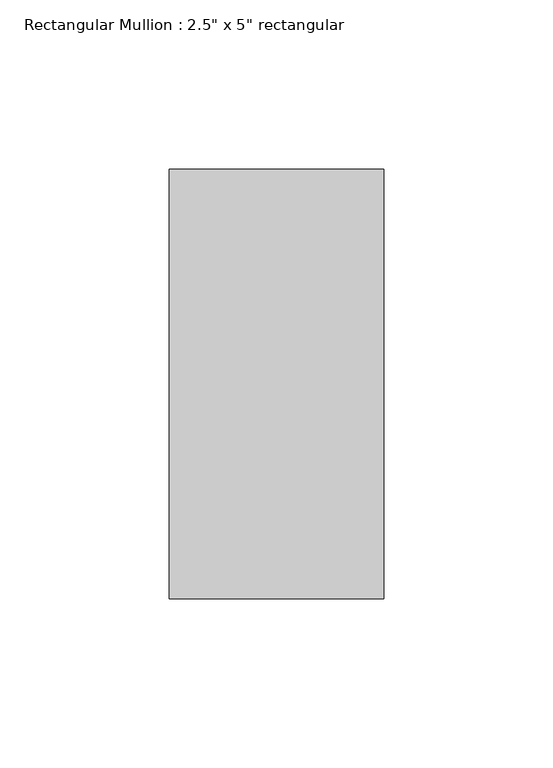
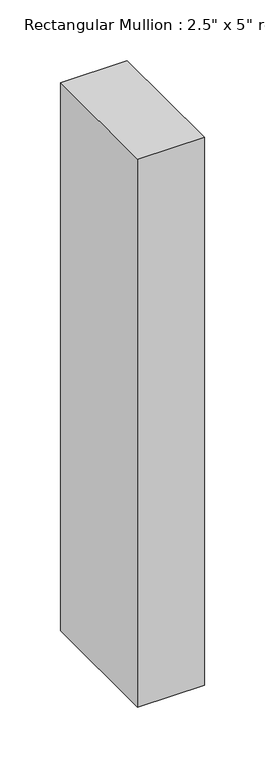
"""IFC4 building model written with IfcOpenShell, lengths in millimetres: member geometry."""

import ifcopenshell
import ifcopenshell.guid

model = None  # the IFC model being written
_history = None  # IfcOwnerHistory: only IFC2X3 demands one
_inside = {}  # id of a spatial element -> (the spatial element, [elements in it])
_under = {}  # id of a project, library or spatial element -> (it, [spatial elements below it])
_declared = {}  # id of a project -> (the project, [libraries it declares])
_typed = {}  # id of a type object -> (the type object, [elements of that type])
_made_of = {}  # id of a material, layer set ... -> (it, [elements and type objects made of it])


def new_model(schema):
    """Start an empty IFC model of exactly this schema.

    Asked for "IFC4X3", IfcOpenShell would pick the latest addendum, in which some entities
    have other attributes; the version numbers below select the first issue.
    IFC2X3 requires an IfcOwnerHistory on every rooted entity: one is made here for all.
    """
    global model, _history
    if schema == "IFC4X3":
        model = ifcopenshell.file(schema_version=(4, 3, 0, 0))
    else:
        model = ifcopenshell.file(schema=schema)
    _inside.clear()
    _under.clear()
    _declared.clear()
    _typed.clear()
    _made_of.clear()
    _history = None
    if model.schema == "IFC2X3":
        org = make("IfcOrganization", Name="unknown")
        user = make(
            "IfcPersonAndOrganization",
            ThePerson=make("IfcPerson", FamilyName="unknown"),
            TheOrganization=org,
        )
        app = make(
            "IfcApplication",
            ApplicationDeveloper=org,
            Version="unknown",
            ApplicationFullName="unknown",
            ApplicationIdentifier="unknown",
        )
        _history = make(
            "IfcOwnerHistory",
            OwningUser=user,
            OwningApplication=app,
            ChangeAction="ADDED",
            CreationDate=0,
        )
    return model


def make(cls, **values):
    """One entity of the class cls with the attributes given. An attribute that is None is left unset."""
    return model.create_entity(
        cls, **{name: value for name, value in values.items() if value is not None}
    )


def rooted(cls, **values):
    """An entity with a GlobalId (a new one), such as an element, a storey or a relation."""
    return make(cls, GlobalId=ifcopenshell.guid.new(), OwnerHistory=_history, **values)


def si_unit(unit_type, name, prefix=None):
    """IfcSIUnit, for example si_unit("LENGTHUNIT", "METRE", prefix="MILLI")."""
    return make("IfcSIUnit", UnitType=unit_type, Prefix=prefix, Name=name)


def assignment(units):
    """IfcUnitAssignment: the units of a project."""
    return None if units is None else make("IfcUnitAssignment", Units=units)


def point(xyz):
    """IfcCartesianPoint."""
    return None if xyz is None else make("IfcCartesianPoint", Coordinates=xyz)


def direction(xyz):
    """IfcDirection."""
    return None if xyz is None else make("IfcDirection", DirectionRatios=xyz)


def frame(location, z_axis=None, x_axis=None):
    """IfcAxis2Placement3D, a coordinate frame: its origin and axes. An axis left out is left unset."""
    return make(
        "IfcAxis2Placement3D",
        Location=point(location),
        Axis=direction(z_axis),
        RefDirection=direction(x_axis),
    )


def origin():
    """The frame at (0, 0, 0) with its axes left unset."""
    return frame((0.0, 0.0, 0.0))


def place(relative_to, where):
    """IfcLocalPlacement: puts the frame where relative to a parent placement (None: the world)."""
    return make(
        "IfcLocalPlacement", PlacementRelTo=relative_to, RelativePlacement=where
    )


def context(
    kind, dimensions, precision=None, world=None, true_north=None, identifier=None
):
    """IfcGeometricRepresentationContext, for example the 3D "Model" context."""
    return make(
        "IfcGeometricRepresentationContext",
        ContextIdentifier=identifier,
        ContextType=kind,
        CoordinateSpaceDimension=dimensions,
        Precision=precision,
        WorldCoordinateSystem=world,
        TrueNorth=true_north,
    )


def project(units=None, contexts=None):
    """IfcProject with its units and contexts."""
    return rooted(
        "IfcProject",
        Name="project",
        RepresentationContexts=contexts,
        UnitsInContext=assignment(units),
    )


def spatial(cls, under=None, at=None, **own):
    """A site, building, storey or space (cls), placed at a placement, below another one or the project."""
    s = rooted(cls, ObjectPlacement=at, **own)
    if under is not None:
        _under.setdefault(under.id(), (under, []))[1].append(s)
    return s


def polyline(points):
    """IfcPolyline through the points."""
    return make("IfcPolyline", Points=[point(p) for p in points])


def outline(outer, holes=None, kind="AREA"):
    """IfcArbitraryClosedProfileDef: a profile drawn as a closed curve; with holes, ...WithVoids."""
    if holes is None:
        return make("IfcArbitraryClosedProfileDef", ProfileType=kind, OuterCurve=outer)
    return make(
        "IfcArbitraryProfileDefWithVoids",
        ProfileType=kind,
        OuterCurve=outer,
        InnerCurves=holes,
    )


def extrude(swept, where, along, depth):
    """IfcExtrudedAreaSolid: the profile swept, set in the frame where, extruded along a direction by depth."""
    return make(
        "IfcExtrudedAreaSolid",
        SweptArea=swept,
        Position=where,
        ExtrudedDirection=direction(along),
        Depth=depth,
    )


def shape(context_of_items, identifier, shape_type, items):
    """IfcShapeRepresentation: the items that make up one representation, for example the "Body"."""
    return make(
        "IfcShapeRepresentation",
        ContextOfItems=context_of_items,
        RepresentationIdentifier=identifier,
        RepresentationType=shape_type,
        Items=items,
    )


def source(mapping_origin, context_of_items, identifier, shape_type, items):
    """IfcRepresentationMap: a shape defined once, which mapped items show again and again."""
    return make(
        "IfcRepresentationMap",
        MappingOrigin=mapping_origin,
        MappedRepresentation=shape(context_of_items, identifier, shape_type, items),
    )


def transform(
    local_origin,
    x_axis=None,
    y_axis=None,
    z_axis=None,
    scale=None,
    scale2=None,
    scale3=None,
    uniform=True,
):
    """IfcCartesianTransformationOperator3D, or its non-uniform kind. x_axis, y_axis, z_axis: its Axis1, 2, 3."""
    if uniform:
        return make(
            "IfcCartesianTransformationOperator3D",
            Axis1=direction(x_axis),
            Axis2=direction(y_axis),
            LocalOrigin=point(local_origin),
            Scale=scale,
            Axis3=direction(z_axis),
        )
    return make(
        "IfcCartesianTransformationOperator3DnonUniform",
        Axis1=direction(x_axis),
        Axis2=direction(y_axis),
        LocalOrigin=point(local_origin),
        Scale=scale,
        Axis3=direction(z_axis),
        Scale2=scale2,
        Scale3=scale3,
    )


def mapped(mapping_source, mapping_target):
    """IfcMappedItem: shows the shape of a source again, moved by a transform."""
    return make(
        "IfcMappedItem", MappingSource=mapping_source, MappingTarget=mapping_target
    )


def made_of(thing, what):
    """Note that an element or type object is made of a material, layer set ...; save() writes the relation."""
    if what is not None:
        _made_of.setdefault(what.id(), (what, []))[1].append(thing)
    return thing


def element(
    cls,
    number,
    at=None,
    inside=None,
    cuts=None,
    type_object=None,
    material=None,
    context=None,
    identifier="Body",
    shape_type=None,
    held_by="IfcProductDefinitionShape",
    body=None,
    shapes=None,
    **own,
):
    """One element of the class cls, such as IfcWall. Its Tag is "e" and its number.

    at: its placement. inside: the storey or other place that contains it. cuts: it is an
    opening in that element (IfcRelVoidsElement). A single representation is given by context,
    identifier, shape_type and body (its items); several are given by shapes. held_by: the class
    of the entity that holds the representations. save() writes the other relations.
    """
    e = rooted(cls, Tag="e%d" % number, ObjectPlacement=at, **own)
    if body is not None:
        shapes = [shape(context, identifier, shape_type, body)]
    if shapes is not None:
        e.Representation = make(held_by, Representations=shapes)
    if inside is not None:
        _inside.setdefault(inside.id(), (inside, []))[1].append(e)
    if cuts is not None:
        rooted(
            "IfcRelVoidsElement", RelatingBuildingElement=cuts, RelatedOpeningElement=e
        )
    if type_object is not None:
        _typed.setdefault(type_object.id(), (type_object, []))[1].append(e)
    return made_of(e, material)


def aggregate(whole, parts):
    """IfcRelAggregates: a whole, such as a stair, and the parts it consists of."""
    return rooted("IfcRelAggregates", RelatingObject=whole, RelatedObjects=parts)


def save(model, path):
    """Write the relations noted so far, then the file.

    IfcRelAggregates (storeys below a building ...), IfcRelContainedInSpatialStructure (elements
    in a storey), IfcRelDefinesByType, IfcRelAssociatesMaterial and IfcRelDeclares: one each for
    every whole, place, type object, material and project.
    """
    for whole, parts in _under.values():
        aggregate(whole, parts)
    for where, things in _inside.values():
        rooted(
            "IfcRelContainedInSpatialStructure",
            RelatedElements=things,
            RelatingStructure=where,
        )
    for kind, things in _typed.values():
        rooted("IfcRelDefinesByType", RelatedObjects=things, RelatingType=kind)
    for what, things in _made_of.values():
        rooted("IfcRelAssociatesMaterial", RelatedObjects=things, RelatingMaterial=what)
    for by, libraries in _declared.values():
        rooted("IfcRelDeclares", RelatingContext=by, RelatedDefinitions=libraries)
    model.write(path)


def member_d5161bba(model_context):
    return source(origin(), model_context, "Body", "SweptSolid", [
        extrude(outline(polyline([(0.0, 63.5), (0.0, -63.5), (-63.5, -63.5), (-63.5, 63.5), (0.0, 63.5)])), frame((0.0, 0.0, -551.035953), z_axis=(0.0, 0.0, 1.0), x_axis=(1.0, 0.0, 0.0)), (0.0, 0.0, 1.0), 551.035953),
    ])


if __name__ == "__main__":
    model = new_model("IFC4")
    model_context = context("Model", 3, world=origin())
    ifc_project = project(units=[si_unit("LENGTHUNIT", "METRE", prefix="MILLI")], contexts=[model_context])
    site = spatial("IfcSite", under=ifc_project)
    building = spatial("IfcBuilding", under=site)
    placement = place(None, origin())
    member_shape = member_d5161bba(model_context)
    element("IfcMember", 1, ObjectType="Rectangular Mullion : 2.5\" x 5\" rectangular", at=placement, inside=building, context=model_context, shape_type="MappedRepresentation", body=[
        mapped(member_shape, transform((0.0, 0.0, 0.0), x_axis=(1.0, 0.0, 0.0), y_axis=(0.0, 1.0, 0.0), z_axis=(0.0, 0.0, 1.0))),
    ])
    save(model, "model.ifc")

# Revit data of these elements
# Type "Rectangular Mullion : 2.5\" x 5\" rectangular"
#   built-in parameter 1007304 = 0.416667 (stored number, unit not read)
#   built-in parameter 1007301 = 0.104167 (stored number, unit not read)
#   built-in parameter 1007300 = 0.104167 (stored number, unit not read)
# Element 1 (IfcMember, "Rectangular Mullion : 2.5\" x 5\" rectangular")
#   Materials on its faces: "Metal - Aluminum 2"
# Materials
#   "Metal - Aluminum 2": class "Metal", colour RGB 189 187 185, transparency 0
